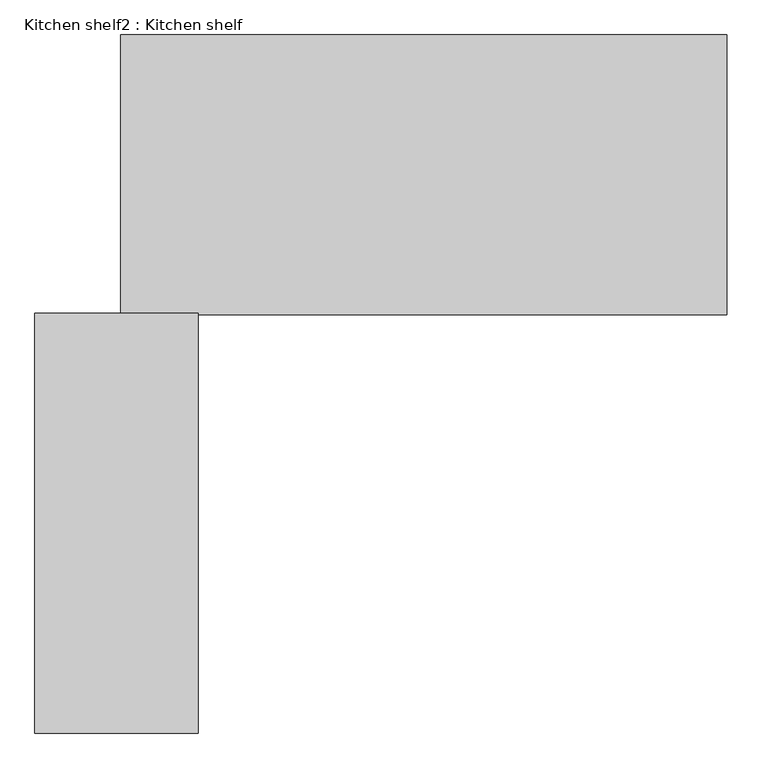
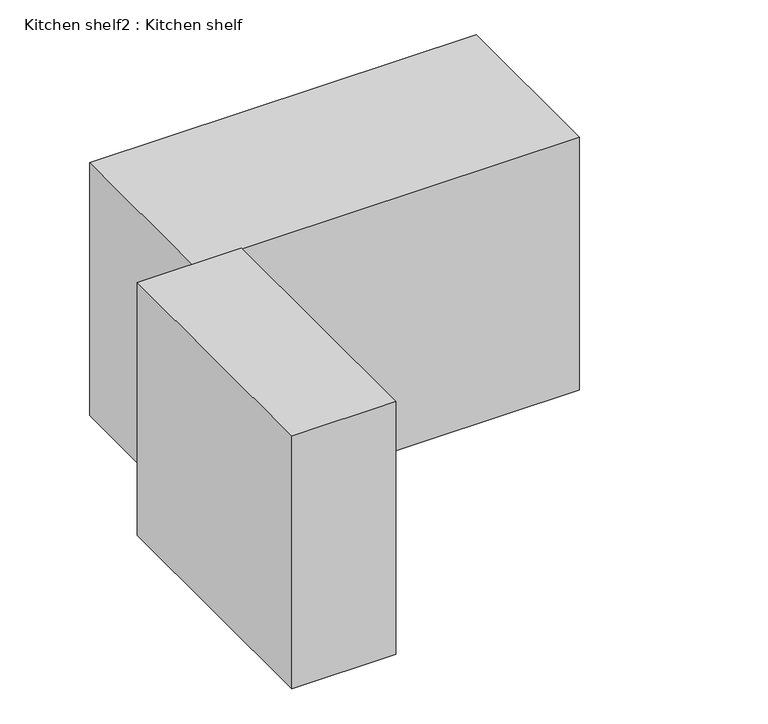
"""IFC4 building model written with IfcOpenShell, lengths in millimetres: furniture geometry, Kitchen shelf2 : Kitchen shelf."""

from ifc_helpers import new_model, si_unit, origin, origin_with_axes, place, context, project, spatial, polyline, outline, extrude, source, transform, mapped, element, save


def kitchen_shelf2_kitchen_shelf_a8e77c75(model_context):
    return source(origin(), model_context, "Body", "SweptSolid", [
        extrude(outline(polyline([(22994.1370052, 10580.3615366), (22994.1370052, 9665.9615366), (22638.5370052, 9665.9615366), (22638.5370052, 10580.3615366), (22994.1370052, 10580.3615366)])), origin_with_axes(), (0.0, 0.0, 1.0), 914.4),
        extrude(outline(polyline([(24146.6620052, 11186.7865366), (24146.6620052, 10577.1865366), (22825.8620052, 10577.1865366), (22825.8620052, 11186.7865366), (24146.6620052, 11186.7865366)])), origin_with_axes(), (0.0, 0.0, 1.0), 914.4),
    ])


if __name__ == "__main__":
    model = new_model("IFC4")
    model_context = context("Model", 3, world=origin())
    ifc_project = project(units=[si_unit("LENGTHUNIT", "METRE", prefix="MILLI")], contexts=[model_context])
    site = spatial("IfcSite", under=ifc_project)
    building = spatial("IfcBuilding", under=site)
    placement = place(None, origin())
    kitchen_shelf2_kitchen_shelf_shape = kitchen_shelf2_kitchen_shelf_a8e77c75(model_context)
    element("IfcFurniture", 1, ObjectType="Kitchen shelf2 : Kitchen shelf", at=placement, inside=building, context=model_context, shape_type="MappedRepresentation", body=[
        mapped(kitchen_shelf2_kitchen_shelf_shape, transform((0.0, 0.0, 0.0), x_axis=(1.0, 0.0, 0.0), y_axis=(0.0, 1.0, 0.0), z_axis=(0.0, 0.0, 1.0))),
    ])
    save(model, "model.ifc")

# Revit data of these elements
# Element 1 (IfcFurniture, "Kitchen shelf2 : Kitchen shelf")
#   Materials on its faces: "food"
# Materials
#   "food": class "Glass", colour RGB 233 233 233, transparency 0, Description = "Soda Lime Glass", Cost = 0
